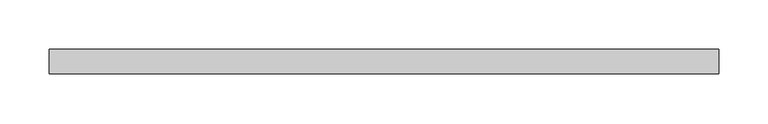
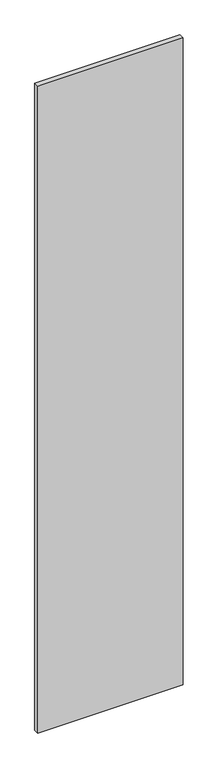
"""IFC4 building model written with IfcOpenShell, lengths in millimetres: plate geometry, 系统嵌板 : 玻璃."""

from ifc_helpers import new_model, si_unit, origin, origin_with_axes, place, context, project, spatial, polyline, outline, extrude, source, transform, mapped, element, save


def plate_e10281fb(model_context):
    return source(origin(), model_context, "Body", "SweptSolid", [
        extrude(outline(polyline([(340.0, -12.5), (-340.0, -12.5), (-340.0, 12.5), (340.0, 12.5), (340.0, -12.5)])), origin_with_axes(), (0.0, 0.0, 1.0), 3200.0),
    ])


if __name__ == "__main__":
    model = new_model("IFC4")
    model_context = context("Model", 3, world=origin())
    ifc_project = project(units=[si_unit("LENGTHUNIT", "METRE", prefix="MILLI")], contexts=[model_context])
    site = spatial("IfcSite", under=ifc_project)
    building = spatial("IfcBuilding", under=site)
    placement = place(None, origin())
    plate_shape = plate_e10281fb(model_context)
    element("IfcPlate", 1, ObjectType="系统嵌板 : 玻璃", at=placement, inside=building, context=model_context, shape_type="MappedRepresentation", body=[
        mapped(plate_shape, transform((0.0, 0.0, 0.0), x_axis=(1.0, 0.0, 0.0), y_axis=(0.0, 1.0, 0.0), z_axis=(0.0, 0.0, 1.0))),
    ])
    save(model, "model.ifc")

# Revit data of these elements
# Type "系统嵌板 : 玻璃"
#   Construction Type Id = "GSP4R"
#   Analytic Construction = "1/8 英寸 Pilkington 单层玻璃"
#   Visual Light Transmittance = 0.9
#   Solar Heat Gain Coefficient = 0.86
#   Heat Transfer Coefficient (U) = 6.7069 W/(m²·K)
# Element 1 (IfcPlate, "系统嵌板 : 玻璃")
#   Materials on its faces: "玻璃"
# Materials
#   "玻璃": class "玻璃", colour RGB 0 128 192, transparency 0.9, Description = "钠钙玻璃", Cost = 0
